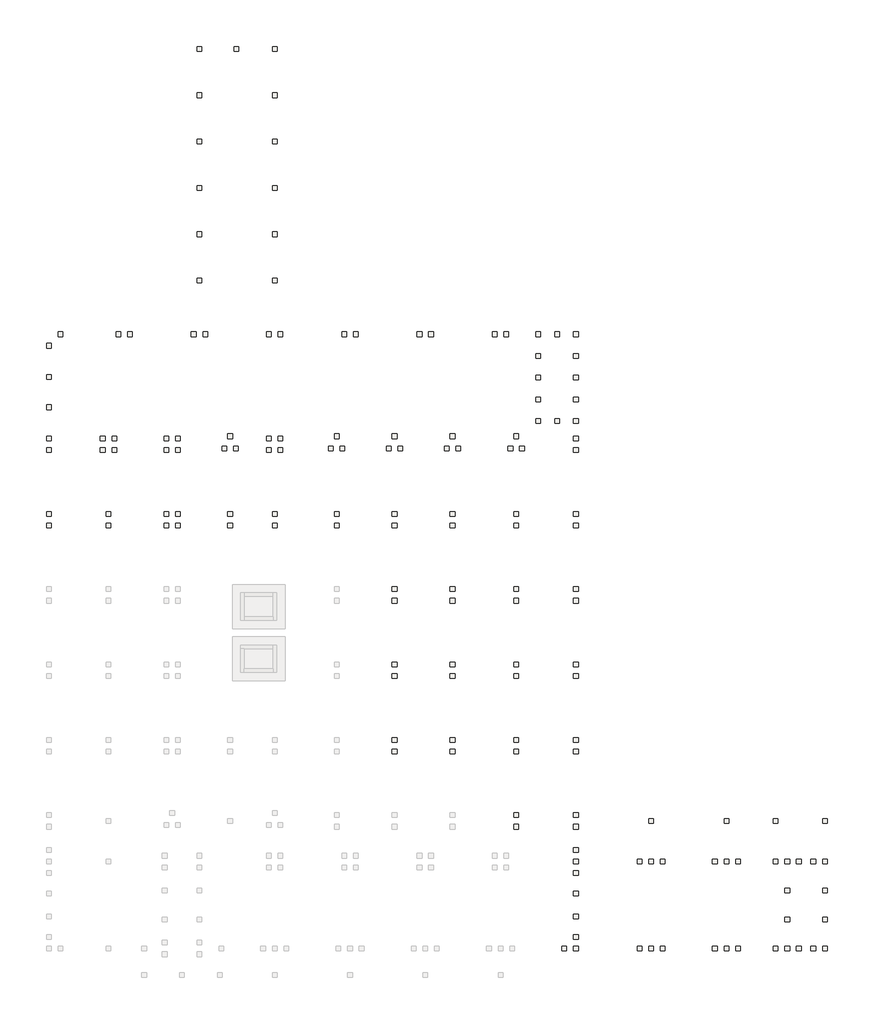
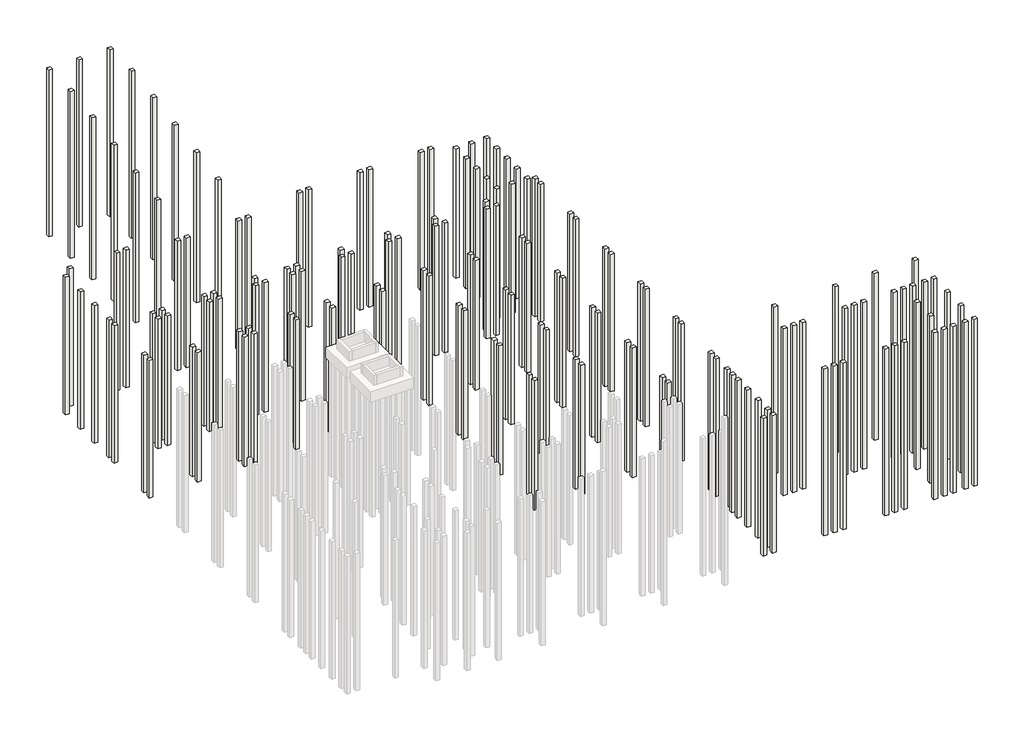
# Not in any storey, part 2 of 2: 160 footings.
# Revit data of these elements (continued)
# Element 4 (IfcFooting, "NLRS_17_SFO_TLB_funderingspaal geheid beton prefab-AV-MMBPC_gen_rsf : heipaal beton prefab_gen__bxh 400x400")
#   IfcGUID = "10$Kfo5uPCAOPJEOo5LEs3"
#   Slanted Angle = 0.00°
#   NLRS_S_draagvermogen_trek = 0.00 kN
#   NLRS_S_draagvermogen_druk = 0.00 kN
#   Angle = 0.00°
#   IsExternal = yes
#   LoadBearing = yes
#   Slanted = 0
#   Phase Created = NLRS_nieuw
#   Materials on its faces: "NLRS_f2_beton prefab_gen_rsf"
# Element 5 (IfcFooting, "NLRS_17_SFO_TLB_funderingspaal geheid beton prefab-AV-MMBPC_gen_rsf : heipaal beton prefab_gen__bxh 400x400")
#   IfcGUID = "10$Kfo5uPCAOPJEOo5LEsU"
#   Slanted Angle = 0.00°
#   NLRS_S_draagvermogen_trek = 0.00 kN
#   NLRS_S_draagvermogen_druk = 0.00 kN
#   Angle = 0.00°
#   IsExternal = yes
#   LoadBearing = yes
#   Slanted = 0
#   Phase Created = NLRS_nieuw
#   Materials on its faces: "NLRS_f2_beton prefab_gen_rsf"
# Element 6 (IfcFooting, "NLRS_17_SFO_TLB_funderingspaal geheid beton prefab-AV-MMBPC_gen_rsf : heipaal beton prefab_gen__bxh 400x400")
#   IfcGUID = "10$Kfo5uPCAOPJEOo5LEsG"
#   Slanted Angle = 0.00°
#   NLRS_S_draagvermogen_trek = 0.00 kN
#   NLRS_S_draagvermogen_druk = 0.00 kN
#   Angle = 0.00°
#   IsExternal = yes
#   LoadBearing = yes
#   Slanted = 0
#   Phase Created = NLRS_nieuw
#   Materials on its faces: "NLRS_f2_beton prefab_gen_rsf"
# Element 7 (IfcFooting, "NLRS_17_SFO_TLB_funderingspaal geheid beton prefab-AV-MMBPC_gen_rsf : heipaal beton prefab_gen__bxh 400x400")
#   IfcGUID = "10$Kfo5uPCAOPJEOo5LEre"
#   Slanted Angle = 0.00°
#   NLRS_S_draagvermogen_trek = 0.00 kN
#   NLRS_S_draagvermogen_druk = 0.00 kN
#   Angle = 0.00°
#   IsExternal = yes
#   LoadBearing = yes
#   Slanted = 0
#   Phase Created = NLRS_nieuw
#   Materials on its faces: "NLRS_f2_beton prefab_gen_rsf"
# Element 8 (IfcFooting, "NLRS_17_SFO_TLB_funderingspaal geheid beton prefab-AV-MMBPC_gen_rsf : heipaal beton prefab_gen__bxh 400x400")
#   IfcGUID = "10$Kfo5uPCAOPJEOo5LErg"
#   Slanted Angle = 0.00°
#   NLRS_S_draagvermogen_trek = 0.00 kN
#   NLRS_S_draagvermogen_druk = 0.00 kN
#   Angle = 0.00°
#   IsExternal = yes
#   LoadBearing = yes
#   Slanted = 0
#   Phase Created = NLRS_nieuw
#   Materials on its faces: "NLRS_f2_beton prefab_gen_rsf"
# Element 9 (IfcFooting, "NLRS_17_SFO_TLB_funderingspaal geheid beton prefab-AV-MMBPC_gen_rsf : heipaal beton prefab_gen__bxh 400x400")
#   IfcGUID = "10$Kfo5uPCAOPJEOo5LEpb"
#   Slanted Angle = 0.00°
#   NLRS_S_draagvermogen_trek = 0.00 kN
#   NLRS_S_draagvermogen_druk = 0.00 kN
#   Angle = 0.00°
#   IsExternal = yes
#   LoadBearing = yes
#   Slanted = 0
#   Phase Created = NLRS_nieuw
#   Materials on its faces: "NLRS_f2_beton prefab_gen_rsf"
# Element 10 (IfcFooting, "NLRS_17_SFO_TLB_funderingspaal geheid beton prefab-AV-MMBPC_gen_rsf : heipaal beton prefab_gen__bxh 400x400")
#   IfcGUID = "10$Kfo5uPCAOPJEOo5LEpd"
#   Slanted Angle = 0.00°
#   NLRS_S_draagvermogen_trek = 0.00 kN
#   NLRS_S_draagvermogen_druk = 0.00 kN
#   Angle = 0.00°
#   IsExternal = yes
#   LoadBearing = yes
#   Slanted = 0
#   Phase Created = NLRS_nieuw
#   Materials on its faces: "NLRS_f2_beton prefab_gen_rsf"
# Element 11 (IfcFooting, "NLRS_17_SFO_TLB_funderingspaal geheid beton prefab-AV-MMBPC_gen_rsf : heipaal beton prefab_gen__bxh 400x400")
#   IfcGUID = "10$Kfo5uPCAOPJEOo5LEpz"
#   Slanted Angle = 0.00°
#   NLRS_S_draagvermogen_trek = 0.00 kN
#   NLRS_S_draagvermogen_druk = 0.00 kN
#   Angle = 0.00°
#   IsExternal = yes
#   LoadBearing = yes
#   Slanted = 0
#   Phase Created = NLRS_nieuw
#   Materials on its faces: "NLRS_f2_beton prefab_gen_rsf"
# Element 12 (IfcFooting, "NLRS_17_SFO_TLB_funderingspaal geheid beton prefab-AV-MMBPC_gen_rsf : heipaal beton prefab_gen__bxh 400x400")
#   IfcGUID = "10$Kfo5uPCAOPJEOo5LEp$"
#   Slanted Angle = 0.00°
#   NLRS_S_draagvermogen_trek = 0.00 kN
#   NLRS_S_draagvermogen_druk = 0.00 kN
#   Angle = 0.00°
#   IsExternal = yes
#   LoadBearing = yes
#   Slanted = 0
#   Phase Created = NLRS_nieuw
#   Materials on its faces: "NLRS_f2_beton prefab_gen_rsf"
# Element 13 (IfcFooting, "NLRS_17_SFO_TLB_funderingspaal geheid beton prefab-AV-MMBPC_gen_rsf : heipaal beton prefab_gen__bxh 400x400")
#   IfcGUID = "10$Kfo5uPCAOPJEOo5LFTh"
#   Slanted Angle = 0.00°
#   NLRS_S_draagvermogen_trek = 0.00 kN
#   NLRS_S_draagvermogen_druk = 0.00 kN
#   Angle = 0.00°
#   IsExternal = yes
#   LoadBearing = yes
#   Slanted = 0
#   Phase Created = NLRS_nieuw
#   Materials on its faces: "NLRS_f2_beton prefab_gen_rsf"
# Element 14 (IfcFooting, "NLRS_17_SFO_TLB_funderingspaal geheid beton prefab-AV-MMBPC_gen_rsf : heipaal beton prefab_gen__bxh 400x400")
#   IfcGUID = "10$Kfo5uPCAOPJEOo5LFSD"
#   Slanted Angle = 0.00°
#   NLRS_S_draagvermogen_trek = 0.00 kN
#   NLRS_S_draagvermogen_druk = 0.00 kN
#   Angle = 0.00°
#   IsExternal = yes
#   LoadBearing = yes
#   Slanted = 0
#   Phase Created = NLRS_nieuw
#   Materials on its faces: "NLRS_f2_beton prefab_gen_rsf"
# Element 15 (IfcFooting, "NLRS_17_SFO_TLB_funderingspaal geheid beton prefab-AV-MMBPC_gen_rsf : heipaal beton prefab_gen__bxh 400x400")
#   IfcGUID = "10$Kfo5uPCAOPJEOo5LFSk"
#   Slanted Angle = 0.00°
#   NLRS_S_draagvermogen_trek = 0.00 kN
#   NLRS_S_draagvermogen_druk = 0.00 kN
#   Angle = 0.00°
#   IsExternal = yes
#   LoadBearing = yes
#   Slanted = 0
#   Phase Created = NLRS_nieuw
#   Materials on its faces: "NLRS_f2_beton prefab_gen_rsf"
# Element 16 (IfcFooting, "NLRS_17_SFO_TLB_funderingspaal geheid beton prefab-AV-MMBPC_gen_rsf : heipaal beton prefab_gen__bxh 400x400")
#   IfcGUID = "10$Kfo5uPCAOPJEOo5LFSv"
#   Slanted Angle = 0.00°
#   NLRS_S_draagvermogen_trek = 0.00 kN
#   NLRS_S_draagvermogen_druk = 0.00 kN
#   Angle = 0.00°
#   IsExternal = yes
#   LoadBearing = yes
#   Slanted = 0
#   Phase Created = NLRS_nieuw
#   Materials on its faces: "NLRS_f2_beton prefab_gen_rsf"
# Element 17 (IfcFooting, "NLRS_17_SFO_TLB_funderingspaal geheid beton prefab-AV-MMBPC_gen_rsf : heipaal beton prefab_gen__bxh 400x400")
#   IfcGUID = "10$Kfo5uPCAOPJEOo5LFSs"
#   Slanted Angle = 0.00°
#   NLRS_S_draagvermogen_trek = 0.00 kN
#   NLRS_S_draagvermogen_druk = 0.00 kN
#   Angle = 0.00°
#   IsExternal = yes
#   LoadBearing = yes
#   Slanted = 0
#   Phase Created = NLRS_nieuw
#   Materials on its faces: "NLRS_f2_beton prefab_gen_rsf"
# Element 18 (IfcFooting, "NLRS_17_SFO_TLB_funderingspaal geheid beton prefab-AV-MMBPC_gen_rsf : heipaal beton prefab_gen__bxh 400x400")
#   IfcGUID = "10$Kfo5uPCAOPJEOo5LFR1"
#   Slanted Angle = 0.00°
#   NLRS_S_draagvermogen_trek = 0.00 kN
#   NLRS_S_draagvermogen_druk = 0.00 kN
#   Angle = 0.00°
#   IsExternal = yes
#   LoadBearing = yes
#   Slanted = 0
#   Phase Created = NLRS_nieuw
#   Materials on its faces: "NLRS_f2_beton prefab_gen_rsf"
# Element 19 (IfcFooting, "NLRS_17_SFO_TLB_funderingspaal geheid beton prefab-AV-MMBPC_gen_rsf : heipaal beton prefab_gen__bxh 400x400")
#   IfcGUID = "10$Kfo5uPCAOPJEOo5LFQO"
#   Slanted Angle = 0.00°
#   NLRS_S_draagvermogen_trek = 0.00 kN
#   NLRS_S_draagvermogen_druk = 0.00 kN
#   Angle = 0.00°
#   IsExternal = yes
#   LoadBearing = yes
#   Slanted = 0
#   Phase Created = NLRS_nieuw
#   Materials on its faces: "NLRS_f2_beton prefab_gen_rsf"
# Element 20 (IfcFooting, "NLRS_17_SFO_TLB_funderingspaal geheid beton prefab-AV-MMBPC_gen_rsf : heipaal beton prefab_gen__bxh 400x400")
#   IfcGUID = "10$Kfo5uPCAOPJEOo5LFQJ"
#   Slanted Angle = 0.00°
#   NLRS_S_draagvermogen_trek = 0.00 kN
#   NLRS_S_draagvermogen_druk = 0.00 kN
#   Angle = 0.00°
#   IsExternal = yes
#   LoadBearing = yes
#   Slanted = 0
#   Phase Created = NLRS_nieuw
#   Materials on its faces: "NLRS_f2_beton prefab_gen_rsf"
# Element 21 (IfcFooting, "NLRS_17_SFO_TLB_funderingspaal geheid beton prefab-AV-MMBPC_gen_rsf : heipaal beton prefab_gen__bxh 400x400")
#   IfcGUID = "10$Kfo5uPCAOPJEOo5LFQk"
#   Slanted Angle = 0.00°
#   NLRS_S_draagvermogen_trek = 0.00 kN
#   NLRS_S_draagvermogen_druk = 0.00 kN
#   Angle = 0.00°
#   IsExternal = yes
#   LoadBearing = yes
#   Slanted = 0
#   Phase Created = NLRS_nieuw
#   Materials on its faces: "NLRS_f2_beton prefab_gen_rsf"
# Element 22 (IfcFooting, "NLRS_17_SFO_TLB_funderingspaal geheid beton prefab-AV-MMBPC_gen_rsf : heipaal beton prefab_gen__bxh 400x400")
#   IfcGUID = "10$Kfo5uPCAOPJEOo5LFPx"
#   Slanted Angle = 0.00°
#   NLRS_S_draagvermogen_trek = 0.00 kN
#   NLRS_S_draagvermogen_druk = 0.00 kN
#   Angle = 0.00°
#   IsExternal = yes
#   LoadBearing = yes
#   Slanted = 0
#   Phase Created = NLRS_nieuw
#   Materials on its faces: "NLRS_f2_beton prefab_gen_rsf"
# Element 23 (IfcFooting, "NLRS_17_SFO_TLB_funderingspaal geheid beton prefab-AV-MMBPC_gen_rsf : heipaal beton prefab_gen__bxh 400x400")
#   IfcGUID = "10$Kfo5uPCAOPJEOo5LFOK"
#   Slanted Angle = 0.00°
#   NLRS_S_draagvermogen_trek = 0.00 kN
#   NLRS_S_draagvermogen_druk = 0.00 kN
#   Angle = 0.00°
#   IsExternal = yes
#   LoadBearing = yes
#   Slanted = 0
#   Phase Created = NLRS_nieuw
#   Materials on its faces: "NLRS_f2_beton prefab_gen_rsf"
# Element 24 (IfcFooting, "NLRS_17_SFO_TLB_funderingspaal geheid beton prefab-AV-MMBPC_gen_rsf : heipaal beton prefab_gen__bxh 400x400")
#   IfcGUID = "10$Kfo5uPCAOPJEOo5LFOl"
#   Slanted Angle = 0.00°
#   NLRS_S_draagvermogen_trek = 0.00 kN
#   NLRS_S_draagvermogen_druk = 0.00 kN
#   Angle = 0.00°
#   IsExternal = yes
#   LoadBearing = yes
#   Slanted = 0
#   Phase Created = NLRS_nieuw
#   Materials on its faces: "NLRS_f2_beton prefab_gen_rsf"
# Element 25 (IfcFooting, "NLRS_17_SFO_TLB_funderingspaal geheid beton prefab-AV-MMBPC_gen_rsf : heipaal beton prefab_gen__bxh 400x400")
#   IfcGUID = "3loy75XKz2Rw4dS8JWiamE"
#   Slanted Angle = 0.00°
#   NLRS_S_draagvermogen_trek = 0.00 kN
#   NLRS_S_draagvermogen_druk = 0.00 kN
#   Angle = 0.00°
#   IsExternal = yes
#   LoadBearing = yes
#   Slanted = 0
#   Phase Created = NLRS_nieuw
#   Materials on its faces: "NLRS_f2_beton prefab_gen_rsf"
# Element 26 (IfcFooting, "NLRS_17_SFO_TLB_funderingspaal geheid beton prefab-AV-MMBPC_gen_rsf : heipaal beton prefab_gen__bxh 400x400")
#   IfcGUID = "3loy75XKz2Rw4dS8JWiamC"
#   Slanted Angle = 0.00°
#   NLRS_S_draagvermogen_trek = 0.00 kN
#   NLRS_S_draagvermogen_druk = 0.00 kN
#   Angle = 0.00°
#   IsExternal = yes
#   LoadBearing = yes
#   Slanted = 0
#   Phase Created = NLRS_nieuw
#   Materials on its faces: "NLRS_f2_beton prefab_gen_rsf"
# Element 27 (IfcFooting, "NLRS_17_SFO_TLB_funderingspaal geheid beton prefab-AV-MMBPC_gen_rsf : heipaal beton prefab_gen__bxh 400x400")
#   IfcGUID = "3loy75XKz2Rw4dS8JWiamv"
#   Slanted Angle = 0.00°
#   NLRS_S_draagvermogen_trek = 0.00 kN
#   NLRS_S_draagvermogen_druk = 0.00 kN
#   Angle = 0.00°
#   IsExternal = yes
#   LoadBearing = yes
#   Slanted = 0
#   Phase Created = NLRS_nieuw
#   Materials on its faces: "NLRS_f2_beton prefab_gen_rsf"
# Element 28 (IfcFooting, "NLRS_17_SFO_TLB_funderingspaal geheid beton prefab-AV-MMBPC_gen_rsf : heipaal beton prefab_gen__bxh 400x400")
#   IfcGUID = "3loy75XKz2Rw4dS8JWiam$"
#   Slanted Angle = 0.00°
#   NLRS_S_draagvermogen_trek = 0.00 kN
#   NLRS_S_draagvermogen_druk = 0.00 kN
#   Angle = 0.00°
#   IsExternal = yes
#   LoadBearing = yes
#   Slanted = 0
#   Phase Created = NLRS_nieuw
#   Materials on its faces: "NLRS_f2_beton prefab_gen_rsf"
# Element 29 (IfcFooting, "NLRS_17_SFO_TLB_funderingspaal geheid beton prefab-AV-MMBPC_gen_rsf : heipaal beton prefab_gen__bxh 400x400")
#   IfcGUID = "3loy75XKz2Rw4dS8JWiama"
#   Slanted Angle = 0.00°
#   NLRS_S_draagvermogen_trek = 0.00 kN
#   NLRS_S_draagvermogen_druk = 0.00 kN
#   Angle = 0.00°
#   IsExternal = yes
#   LoadBearing = yes
#   Slanted = 0
#   Phase Created = NLRS_nieuw
#   Materials on its faces: "NLRS_f2_beton prefab_gen_rsf"
# Element 30 (IfcFooting, "NLRS_17_SFO_TLB_funderingspaal geheid beton prefab-AV-MMBPC_gen_rsf : heipaal beton prefab_gen__bxh 400x400")
#   IfcGUID = "3loy75XKz2Rw4dS8JWiamg"
#   Slanted Angle = 0.00°
#   NLRS_S_draagvermogen_trek = 0.00 kN
#   NLRS_S_draagvermogen_druk = 0.00 kN
#   Angle = 0.00°
#   IsExternal = yes
#   LoadBearing = yes
#   Slanted = 0
#   Phase Created = NLRS_nieuw
#   Materials on its faces: "NLRS_f2_beton prefab_gen_rsf"
# Element 31 (IfcFooting, "NLRS_17_SFO_TLB_funderingspaal geheid beton prefab-AV-MMBPC_gen_rsf : heipaal beton prefab_gen__bxh 400x400")
#   IfcGUID = "3loy75XKz2Rw4dS8JWiapN"
#   Slanted Angle = 0.00°
#   NLRS_S_draagvermogen_trek = 0.00 kN
#   NLRS_S_draagvermogen_druk = 0.00 kN
#   Angle = 0.00°
#   IsExternal = yes
#   LoadBearing = yes
#   Slanted = 0
#   Phase Created = NLRS_nieuw
#   Materials on its faces: "NLRS_f2_beton prefab_gen_rsf"
# Element 32 (IfcFooting, "NLRS_17_SFO_TLB_funderingspaal geheid beton prefab-AV-MMBPC_gen_rsf : heipaal beton prefab_gen__bxh 400x400")
#   IfcGUID = "3loy75XKz2Rw4dS8JWiapL"
#   Slanted Angle = 0.00°
#   NLRS_S_draagvermogen_trek = 0.00 kN
#   NLRS_S_draagvermogen_druk = 0.00 kN
#   Angle = 0.00°
#   IsExternal = yes
#   LoadBearing = yes
#   Slanted = 0
#   Phase Created = NLRS_nieuw
#   Materials on its faces: "NLRS_f2_beton prefab_gen_rsf"
# Element 33 (IfcFooting, "NLRS_17_SFO_TLB_funderingspaal geheid beton prefab-AV-MMBPC_gen_rsf : heipaal beton prefab_gen__bxh 400x400")
#   IfcGUID = "3loy75XKz2Rw4dS8JWiap2"
#   Slanted Angle = 0.00°
#   NLRS_S_draagvermogen_trek = 0.00 kN
#   NLRS_S_draagvermogen_druk = 0.00 kN
#   Angle = 0.00°
#   IsExternal = yes
#   LoadBearing = yes
#   Slanted = 0
#   Phase Created = NLRS_nieuw
#   Materials on its faces: "NLRS_f2_beton prefab_gen_rsf"
# Element 34 (IfcFooting, "NLRS_17_SFO_TLB_funderingspaal geheid beton prefab-AV-MMBPC_gen_rsf : heipaal beton prefab_gen__bxh 400x400")
#   IfcGUID = "3loy75XKz2Rw4dS8JWiap0"
#   Slanted Angle = 0.00°
#   NLRS_S_draagvermogen_trek = 0.00 kN
#   NLRS_S_draagvermogen_druk = 0.00 kN
#   Angle = 0.00°
#   IsExternal = yes
#   LoadBearing = yes
#   Slanted = 0
#   Phase Created = NLRS_nieuw
#   Materials on its faces: "NLRS_f2_beton prefab_gen_rsf"
# Element 35 (IfcFooting, "NLRS_17_SFO_TLB_funderingspaal geheid beton prefab-AV-MMBPC_gen_rsf : heipaal beton prefab_gen__bxh 400x400")
#   IfcGUID = "3loy75XKz2Rw4dS8JWiapD"
#   Slanted Angle = 0.00°
#   NLRS_S_draagvermogen_trek = 0.00 kN
#   NLRS_S_draagvermogen_druk = 0.00 kN
#   Angle = 0.00°
#   IsExternal = yes
#   LoadBearing = yes
#   Slanted = 0
#   Phase Created = NLRS_nieuw
#   Materials on its faces: "NLRS_f2_beton prefab_gen_rsf"
# Element 36 (IfcFooting, "NLRS_17_SFO_TLB_funderingspaal geheid beton prefab-AV-MMBPC_gen_rsf : heipaal beton prefab_gen__bxh 400x400")
#   IfcGUID = "3loy75XKz2Rw4dS8JWiapp"
#   Slanted Angle = 0.00°
#   NLRS_S_draagvermogen_trek = 0.00 kN
#   NLRS_S_draagvermogen_druk = 0.00 kN
#   Angle = 0.00°
#   IsExternal = yes
#   LoadBearing = yes
#   Slanted = 0
#   Phase Created = NLRS_nieuw
#   Materials on its faces: "NLRS_f2_beton prefab_gen_rsf"
# Element 37 (IfcFooting, "NLRS_17_SFO_TLB_funderingspaal geheid beton prefab-AV-MMBPC_gen_rsf : heipaal beton prefab_gen__bxh 400x400")
#   IfcGUID = "3loy75XKz2Rw4dS8JWiao6"
#   Slanted Angle = 0.00°
#   NLRS_S_draagvermogen_trek = 0.00 kN
#   NLRS_S_draagvermogen_druk = 0.00 kN
#   Angle = 0.00°
#   IsExternal = yes
#   LoadBearing = yes
#   Slanted = 0
#   Phase Created = NLRS_nieuw
#   Materials on its faces: "NLRS_f2_beton prefab_gen_rsf"
# Element 38 (IfcFooting, "NLRS_17_SFO_TLB_funderingspaal geheid beton prefab-AV-MMBPC_gen_rsf : heipaal beton prefab_gen__bxh 400x400")
#   IfcGUID = "3loy75XKz2Rw4dS8JWiao4"
#   Slanted Angle = 0.00°
#   NLRS_S_draagvermogen_trek = 0.00 kN
#   NLRS_S_draagvermogen_druk = 0.00 kN
#   Angle = 0.00°
#   IsExternal = yes
#   LoadBearing = yes
#   Slanted = 0
#   Phase Created = NLRS_nieuw
#   Materials on its faces: "NLRS_f2_beton prefab_gen_rsf"
# Element 39 (IfcFooting, "NLRS_17_SFO_TLB_funderingspaal geheid beton prefab-AV-MMBPC_gen_rsf : heipaal beton prefab_gen__bxh 400x400")
#   IfcGUID = "3loy75XKz2Rw4dS8JWiaon"
#   Slanted Angle = 0.00°
#   NLRS_S_draagvermogen_trek = 0.00 kN
#   NLRS_S_draagvermogen_druk = 0.00 kN
#   Angle = 0.00°
#   IsExternal = yes
#   LoadBearing = yes
#   Slanted = 0
#   Phase Created = NLRS_nieuw
#   Materials on its faces: "NLRS_f2_beton prefab_gen_rsf"
# Element 40 (IfcFooting, "NLRS_17_SFO_TLB_funderingspaal geheid beton prefab-AV-MMBPC_gen_rsf : heipaal beton prefab_gen__bxh 400x400")
#   IfcGUID = "3loy75XKz2Rw4dS8JWiaot"
#   Slanted Angle = 0.00°
#   NLRS_S_draagvermogen_trek = 0.00 kN
#   NLRS_S_draagvermogen_druk = 0.00 kN
#   Angle = 0.00°
#   IsExternal = yes
#   LoadBearing = yes
#   Slanted = 0
#   Phase Created = NLRS_nieuw
#   Materials on its faces: "NLRS_f2_beton prefab_gen_rsf"
# Element 41 (IfcFooting, "NLRS_17_SFO_TLB_funderingspaal geheid beton prefab-AV-MMBPC_gen_rsf : heipaal beton prefab_gen__bxh 400x400")
#   IfcGUID = "3loy75XKz2Rw4dS8JWiaoy"
#   Slanted Angle = 0.00°
#   NLRS_S_draagvermogen_trek = 0.00 kN
#   NLRS_S_draagvermogen_druk = 0.00 kN
#   Angle = 0.00°
#   IsExternal = yes
#   LoadBearing = yes
#   Slanted = 0
#   Phase Created = NLRS_nieuw
#   Materials on its faces: "NLRS_f2_beton prefab_gen_rsf"
# Element 42 (IfcFooting, "NLRS_17_SFO_TLB_funderingspaal geheid beton prefab-AV-MMBPC_gen_rsf : heipaal beton prefab_gen__bxh 400x400")
#   IfcGUID = "3loy75XKz2Rw4dS8JWiaoY"
#   Slanted Angle = 0.00°
#   NLRS_S_draagvermogen_trek = 0.00 kN
#   NLRS_S_draagvermogen_druk = 0.00 kN
#   Angle = 0.00°
#   IsExternal = yes
#   LoadBearing = yes
#   Slanted = 0
#   Phase Created = NLRS_nieuw
#   Materials on its faces: "NLRS_f2_beton prefab_gen_rsf"
# Element 43 (IfcFooting, "NLRS_17_SFO_TLB_funderingspaal geheid beton prefab-AV-MMBPC_gen_rsf : heipaal beton prefab_gen__bxh 400x400")
#   IfcGUID = "3loy75XKz2Rw4dS8JWiaol"
#   Slanted Angle = 0.00°
#   NLRS_S_draagvermogen_trek = 0.00 kN
#   NLRS_S_draagvermogen_druk = 0.00 kN
#   Angle = 0.00°
#   IsExternal = yes
#   LoadBearing = yes
#   Slanted = 0
#   Phase Created = NLRS_nieuw
#   Materials on its faces: "NLRS_f2_beton prefab_gen_rsf"
# Element 44 (IfcFooting, "NLRS_17_SFO_TLB_funderingspaal geheid beton prefab-AV-MMBPC_gen_rsf : heipaal beton prefab_gen__bxh 400x400")
#   IfcGUID = "3loy75XKz2Rw4dS8JWiaoj"
#   Slanted Angle = 0.00°
#   NLRS_S_draagvermogen_trek = 0.00 kN
#   NLRS_S_draagvermogen_druk = 0.00 kN
#   Angle = 0.00°
#   IsExternal = yes
#   LoadBearing = yes
#   Slanted = 0
#   Phase Created = NLRS_nieuw
#   Materials on its faces: "NLRS_f2_beton prefab_gen_rsf"
# Element 45 (IfcFooting, "NLRS_17_SFO_TLB_funderingspaal geheid beton prefab-AV-MMBPC_gen_rsf : heipaal beton prefab_gen__bxh 400x400")
#   IfcGUID = "3loy75XKz2Rw4dS8JWiarQ"
#   Slanted Angle = 0.00°
#   NLRS_S_draagvermogen_trek = 0.00 kN
#   NLRS_S_draagvermogen_druk = 0.00 kN
#   Angle = 0.00°
#   IsExternal = yes
#   LoadBearing = yes
#   Slanted = 0
#   Phase Created = NLRS_nieuw
#   Materials on its faces: "NLRS_f2_beton prefab_gen_rsf"
# Element 46 (IfcFooting, "NLRS_17_SFO_TLB_funderingspaal geheid beton prefab-AV-MMBPC_gen_rsf : heipaal beton prefab_gen__bxh 400x400")
#   IfcGUID = "3loy75XKz2Rw4dS8JWiarO"
#   Slanted Angle = 0.00°
#   NLRS_S_draagvermogen_trek = 0.00 kN
#   NLRS_S_draagvermogen_druk = 0.00 kN
#   Angle = 0.00°
#   IsExternal = yes
#   LoadBearing = yes
#   Slanted = 0
#   Phase Created = NLRS_nieuw
#   Materials on its faces: "NLRS_f2_beton prefab_gen_rsf"
# Element 47 (IfcFooting, "NLRS_17_SFO_TLB_funderingspaal geheid beton prefab-AV-MMBPC_gen_rsf : heipaal beton prefab_gen__bxh 400x400")
#   IfcGUID = "3loy75XKz2Rw4dS8JWiar5"
#   Slanted Angle = 0.00°
#   NLRS_S_draagvermogen_trek = 0.00 kN
#   NLRS_S_draagvermogen_druk = 0.00 kN
#   Angle = 0.00°
#   IsExternal = yes
#   LoadBearing = yes
#   Slanted = 0
#   Phase Created = NLRS_nieuw
#   Materials on its faces: "NLRS_f2_beton prefab_gen_rsf"
# Element 48 (IfcFooting, "NLRS_17_SFO_TLB_funderingspaal geheid beton prefab-AV-MMBPC_gen_rsf : heipaal beton prefab_gen__bxh 400x400")
#   IfcGUID = "3loy75XKz2Rw4dS8JWiarB"
#   Slanted Angle = 0.00°
#   NLRS_S_draagvermogen_trek = 0.00 kN
#   NLRS_S_draagvermogen_druk = 0.00 kN
#   Angle = 0.00°
#   IsExternal = yes
#   LoadBearing = yes
#   Slanted = 0
#   Phase Created = NLRS_nieuw
#   Materials on its faces: "NLRS_f2_beton prefab_gen_rsf"
# Element 49 (IfcFooting, "NLRS_17_SFO_TLB_funderingspaal geheid beton prefab-AV-MMBPC_gen_rsf : heipaal beton prefab_gen__bxh 400x400")
#   IfcGUID = "3loy75XKz2Rw4dS8JWiarm"
#   Slanted Angle = 0.00°
#   NLRS_S_draagvermogen_trek = 0.00 kN
#   NLRS_S_draagvermogen_druk = 0.00 kN
#   Angle = 0.00°
#   IsExternal = yes
#   LoadBearing = yes
#   Slanted = 0
#   Phase Created = NLRS_nieuw
#   Materials on its faces: "NLRS_f2_beton prefab_gen_rsf"
# Element 50 (IfcFooting, "NLRS_17_SFO_TLB_funderingspaal geheid beton prefab-AV-MMBPC_gen_rsf : heipaal beton prefab_gen__bxh 400x400")
#   IfcGUID = "3loy75XKz2Rw4dS8JWiars"
#   Slanted Angle = 0.00°
#   NLRS_S_draagvermogen_trek = 0.00 kN
#   NLRS_S_draagvermogen_druk = 0.00 kN
#   Angle = 0.00°
#   IsExternal = yes
#   LoadBearing = yes
#   Slanted = 0
#   Phase Created = NLRS_nieuw
#   Materials on its faces: "NLRS_f2_beton prefab_gen_rsf"
# Element 51 (IfcFooting, "NLRS_17_SFO_TLB_funderingspaal geheid beton prefab-AV-MMBPC_gen_rsf : heipaal beton prefab_gen__bxh 400x400")
#   IfcGUID = "3loy75XKz2Rw4dS8JWia96"
#   Slanted Angle = 0.00°
#   NLRS_S_draagvermogen_trek = 0.00 kN
#   NLRS_S_draagvermogen_druk = 0.00 kN
#   Angle = 0.00°
#   IsExternal = yes
#   LoadBearing = yes
#   Slanted = 0
#   Phase Created = NLRS_nieuw
#   Materials on its faces: "NLRS_f2_beton prefab_gen_rsf"
# Element 52 (IfcFooting, "NLRS_17_SFO_TLB_funderingspaal geheid beton prefab-AV-MMBPC_gen_rsf : heipaal beton prefab_gen__bxh 400x400")
#   IfcGUID = "3loy75XKz2Rw4dS8JWia94"
#   Slanted Angle = 0.00°
#   NLRS_S_draagvermogen_trek = 0.00 kN
#   NLRS_S_draagvermogen_druk = 0.00 kN
#   Angle = 0.00°
#   IsExternal = yes
#   LoadBearing = yes
#   Slanted = 0
#   Phase Created = NLRS_nieuw
#   Materials on its faces: "NLRS_f2_beton prefab_gen_rsf"
# Element 53 (IfcFooting, "NLRS_17_SFO_TLB_funderingspaal geheid beton prefab-AV-MMBPC_gen_rsf : heipaal beton prefab_gen__bxh 400x400")
#   IfcGUID = "3loy75XKz2Rw4dS8JWia9A"
#   Slanted Angle = 0.00°
#   NLRS_S_draagvermogen_trek = 0.00 kN
#   NLRS_S_draagvermogen_druk = 0.00 kN
#   Angle = 0.00°
#   IsExternal = yes
#   LoadBearing = yes
#   Slanted = 0
#   Phase Created = NLRS_nieuw
#   Materials on its faces: "NLRS_f2_beton prefab_gen_rsf"
# Element 54 (IfcFooting, "NLRS_17_SFO_TLB_funderingspaal geheid beton prefab-AV-MMBPC_gen_rsf : heipaal beton prefab_gen__bxh 400x400")
#   IfcGUID = "3loy75XKz2Rw4dS8JWia98"
#   Slanted Angle = 0.00°
#   NLRS_S_draagvermogen_trek = 0.00 kN
#   NLRS_S_draagvermogen_druk = 0.00 kN
#   Angle = 0.00°
#   IsExternal = yes
#   LoadBearing = yes
#   Slanted = 0
#   Phase Created = NLRS_nieuw
#   Materials on its faces: "NLRS_f2_beton prefab_gen_rsf"
# Element 55 (IfcFooting, "NLRS_17_SFO_TLB_funderingspaal geheid beton prefab-AV-MMBPC_gen_rsf : heipaal beton prefab_gen__bxh 400x400")
#   IfcGUID = "3loy75XKz2Rw4dS8JWia9l"
#   Slanted Angle = 0.00°
#   NLRS_S_draagvermogen_trek = 0.00 kN
#   NLRS_S_draagvermogen_druk = 0.00 kN
#   Angle = 0.00°
#   IsExternal = yes
#   LoadBearing = yes
#   Slanted = 0
#   Phase Created = NLRS_nieuw
#   Materials on its faces: "NLRS_f2_beton prefab_gen_rsf"
# Element 56 (IfcFooting, "NLRS_17_SFO_TLB_funderingspaal geheid beton prefab-AV-MMBPC_gen_rsf : heipaal beton prefab_gen__bxh 400x400")
#   IfcGUID = "3loy75XKz2Rw4dS8JWia9j"
#   Slanted Angle = 0.00°
#   NLRS_S_draagvermogen_trek = 0.00 kN
#   NLRS_S_draagvermogen_druk = 0.00 kN
#   Angle = 0.00°
#   IsExternal = yes
#   LoadBearing = yes
#   Slanted = 0
#   Phase Created = NLRS_nieuw
#   Materials on its faces: "NLRS_f2_beton prefab_gen_rsf"
# Element 57 (IfcFooting, "NLRS_17_SFO_TLB_funderingspaal geheid beton prefab-AV-MMBPC_gen_rsf : heipaal beton prefab_gen__bxh 400x400")
#   IfcGUID = "3loy75XKz2Rw4dS8JWia8J"
#   Slanted Angle = 0.00°
#   NLRS_S_draagvermogen_trek = 0.00 kN
#   NLRS_S_draagvermogen_druk = 0.00 kN
#   Angle = 0.00°
#   IsExternal = yes
#   LoadBearing = yes
#   Slanted = 0
#   Phase Created = NLRS_nieuw
#   Materials on its faces: "NLRS_f2_beton prefab_gen_rsf"
# Element 58 (IfcFooting, "NLRS_17_SFO_TLB_funderingspaal geheid beton prefab-AV-MMBPC_gen_rsf : heipaal beton prefab_gen__bxh 400x400")
#   IfcGUID = "3loy75XKz2Rw4dS8JWia8H"
#   Slanted Angle = 0.00°
#   NLRS_S_draagvermogen_trek = 0.00 kN
#   NLRS_S_draagvermogen_druk = 0.00 kN
#   Angle = 0.00°
#   IsExternal = yes
#   LoadBearing = yes
#   Slanted = 0
#   Phase Created = NLRS_nieuw
#   Materials on its faces: "NLRS_f2_beton prefab_gen_rsf"
# Element 59 (IfcFooting, "NLRS_17_SFO_TLB_funderingspaal geheid beton prefab-AV-MMBPC_gen_rsf : heipaal beton prefab_gen__bxh 400x400")
#   IfcGUID = "3loy75XKz2Rw4dS8JWia8q"
#   Slanted Angle = 0.00°
#   NLRS_S_draagvermogen_trek = 0.00 kN
#   NLRS_S_draagvermogen_druk = 0.00 kN
#   Angle = 0.00°
#   IsExternal = yes
#   LoadBearing = yes
#   Slanted = 0
#   Phase Created = NLRS_nieuw
#   Materials on its faces: "NLRS_f2_beton prefab_gen_rsf"
# Element 60 (IfcFooting, "NLRS_17_SFO_TLB_funderingspaal geheid beton prefab-AV-MMBPC_gen_rsf : heipaal beton prefab_gen__bxh 400x400")
#   IfcGUID = "3loy75XKz2Rw4dS8JWia8w"
#   Slanted Angle = 0.00°
#   NLRS_S_draagvermogen_trek = 0.00 kN
#   NLRS_S_draagvermogen_druk = 0.00 kN
#   Angle = 0.00°
#   IsExternal = yes
#   LoadBearing = yes
#   Slanted = 0
#   Phase Created = NLRS_nieuw
#   Materials on its faces: "NLRS_f2_beton prefab_gen_rsf"
# Element 61 (IfcFooting, "NLRS_17_SFO_TLB_funderingspaal geheid beton prefab-AV-MMBPC_gen_rsf : heipaal beton prefab_gen__bxh 400x400")
#   IfcGUID = "3loy75XKz2Rw4dS8JWia8u"
#   Slanted Angle = 0.00°
#   NLRS_S_draagvermogen_trek = 0.00 kN
#   NLRS_S_draagvermogen_druk = 0.00 kN
#   Angle = 0.00°
#   IsExternal = yes
#   LoadBearing = yes
#   Slanted = 0
#   Phase Created = NLRS_nieuw
#   Materials on its faces: "NLRS_f2_beton prefab_gen_rsf"
# Element 62 (IfcFooting, "NLRS_17_SFO_TLB_funderingspaal geheid beton prefab-AV-MMBPC_gen_rsf : heipaal beton prefab_gen__bxh 400x400")
#   IfcGUID = "3loy75XKz2Rw4dS8JWiaDh"
#   Slanted Angle = 0.00°
#   NLRS_S_draagvermogen_trek = 0.00 kN
#   NLRS_S_draagvermogen_druk = 0.00 kN
#   Angle = 0.00°
#   IsExternal = yes
#   LoadBearing = yes
#   Slanted = 0
#   Phase Created = NLRS_nieuw
#   Materials on its faces: "NLRS_f2_beton prefab_gen_rsf"
# Element 63 (IfcFooting, "NLRS_17_SFO_TLB_funderingspaal geheid beton prefab-AV-MMBPC_gen_rsf : heipaal beton prefab_gen__bxh 400x400")
#   IfcGUID = "3loy75XKz2Rw4dS8JWiaDf"
#   Slanted Angle = 0.00°
#   NLRS_S_draagvermogen_trek = 0.00 kN
#   NLRS_S_draagvermogen_druk = 0.00 kN
#   Angle = 0.00°
#   IsExternal = yes
#   LoadBearing = yes
#   Slanted = 0
#   Phase Created = NLRS_nieuw
#   Materials on its faces: "NLRS_f2_beton prefab_gen_rsf"
# Element 64 (IfcFooting, "NLRS_17_SFO_TLB_funderingspaal geheid beton prefab-AV-MMBPC_gen_rsf : heipaal beton prefab_gen__bxh 400x400")
#   IfcGUID = "3loy75XKz2Rw4dS8JWiaDl"
#   Slanted Angle = 0.00°
#   NLRS_S_draagvermogen_trek = 0.00 kN
#   NLRS_S_draagvermogen_druk = 0.00 kN
#   Angle = 0.00°
#   IsExternal = yes
#   LoadBearing = yes
#   Slanted = 0
#   Phase Created = NLRS_nieuw
#   Materials on its faces: "NLRS_f2_beton prefab_gen_rsf"
# Element 65 (IfcFooting, "NLRS_17_SFO_TLB_funderingspaal geheid beton prefab-AV-MMBPC_gen_rsf : heipaal beton prefab_gen__bxh 400x400")
#   IfcGUID = "3loy75XKz2Rw4dS8JWiaDj"
#   Slanted Angle = 0.00°
#   NLRS_S_draagvermogen_trek = 0.00 kN
#   NLRS_S_draagvermogen_druk = 0.00 kN
#   Angle = 0.00°
#   IsExternal = yes
#   LoadBearing = yes
#   Slanted = 0
#   Phase Created = NLRS_nieuw
#   Materials on its faces: "NLRS_f2_beton prefab_gen_rsf"
# Element 66 (IfcFooting, "NLRS_17_SFO_TLB_funderingspaal geheid beton prefab-AV-MMBPC_gen_rsf : heipaal beton prefab_gen__bxh 400x400")
#   IfcGUID = "3loy75XKz2Rw4dS8JWiaC7"
#   Slanted Angle = 0.00°
#   NLRS_S_draagvermogen_trek = 0.00 kN
#   NLRS_S_draagvermogen_druk = 0.00 kN
#   Angle = 0.00°
#   IsExternal = yes
#   LoadBearing = yes
#   Slanted = 0
#   Phase Created = NLRS_nieuw
#   Materials on its faces: "NLRS_f2_beton prefab_gen_rsf"
# Element 67 (IfcFooting, "NLRS_17_SFO_TLB_funderingspaal geheid beton prefab-AV-MMBPC_gen_rsf : heipaal beton prefab_gen__bxh 400x400")
#   IfcGUID = "3loy75XKz2Rw4dS8JWiaC5"
#   Slanted Angle = 0.00°
#   NLRS_S_draagvermogen_trek = 0.00 kN
#   NLRS_S_draagvermogen_druk = 0.00 kN
#   Angle = 0.00°
#   IsExternal = yes
#   LoadBearing = yes
#   Slanted = 0
#   Phase Created = NLRS_nieuw
#   Materials on its faces: "NLRS_f2_beton prefab_gen_rsf"
# Element 68 (IfcFooting, "NLRS_17_SFO_TLB_funderingspaal geheid beton prefab-AV-MMBPC_gen_rsf : heipaal beton prefab_gen__bxh 400x400")
#   IfcGUID = "3loy75XKz2Rw4dS8JWiaCB"
#   Slanted Angle = 0.00°
#   NLRS_S_draagvermogen_trek = 0.00 kN
#   NLRS_S_draagvermogen_druk = 0.00 kN
#   Angle = 0.00°
#   IsExternal = yes
#   LoadBearing = yes
#   Slanted = 0
#   Phase Created = NLRS_nieuw
#   Materials on its faces: "NLRS_f2_beton prefab_gen_rsf"
# Element 69 (IfcFooting, "NLRS_17_SFO_TLB_funderingspaal geheid beton prefab-AV-MMBPC_gen_rsf : heipaal beton prefab_gen__bxh 400x400")
#   IfcGUID = "3loy75XKz2Rw4dS8JWiaCs"
#   Slanted Angle = 0.00°
#   NLRS_S_draagvermogen_trek = 0.00 kN
#   NLRS_S_draagvermogen_druk = 0.00 kN
#   Angle = 0.00°
#   IsExternal = yes
#   LoadBearing = yes
#   Slanted = 0
#   Phase Created = NLRS_nieuw
#   Materials on its faces: "NLRS_f2_beton prefab_gen_rsf"
# Element 70 (IfcFooting, "NLRS_17_SFO_TLB_funderingspaal geheid beton prefab-AV-MMBPC_gen_rsf : heipaal beton prefab_gen__bxh 400x400")
#   IfcGUID = "3loy75XKz2Rw4dS8JWiaCq"
#   Slanted Angle = 0.00°
#   NLRS_S_draagvermogen_trek = 0.00 kN
#   NLRS_S_draagvermogen_druk = 0.00 kN
#   Angle = 0.00°
#   IsExternal = yes
#   LoadBearing = yes
#   Slanted = 0
#   Phase Created = NLRS_nieuw
#   Materials on its faces: "NLRS_f2_beton prefab_gen_rsf"
# Element 71 (IfcFooting, "NLRS_17_SFO_TLB_funderingspaal geheid beton prefab-AV-MMBPC_gen_rsf : heipaal beton prefab_gen__bxh 400x400")
#   IfcGUID = "3loy75XKz2Rw4dS8JWiaCw"
#   Slanted Angle = 0.00°
#   NLRS_S_draagvermogen_trek = 0.00 kN
#   NLRS_S_draagvermogen_druk = 0.00 kN
#   Angle = 0.00°
#   IsExternal = yes
#   LoadBearing = yes
#   Slanted = 0
#   Phase Created = NLRS_nieuw
#   Materials on its faces: "NLRS_f2_beton prefab_gen_rsf"
# Element 72 (IfcFooting, "NLRS_17_SFO_TLB_funderingspaal geheid beton prefab-AV-MMBPC_gen_rsf : heipaal beton prefab_gen__bxh 400x400")
#   IfcGUID = "3loy75XKz2Rw4dS8JWiaCb"
#   Slanted Angle = 0.00°
#   NLRS_S_draagvermogen_trek = 0.00 kN
#   NLRS_S_draagvermogen_druk = 0.00 kN
#   Angle = 0.00°
#   IsExternal = yes
#   LoadBearing = yes
#   Slanted = 0
#   Phase Created = NLRS_nieuw
#   Materials on its faces: "NLRS_f2_beton prefab_gen_rsf"
# Element 73 (IfcFooting, "NLRS_17_SFO_TLB_funderingspaal geheid beton prefab-AV-MMBPC_gen_rsf : heipaal beton prefab_gen__bxh 400x400")
#   IfcGUID = "3loy75XKz2Rw4dS8JWiaCh"
#   Slanted Angle = 0.00°
#   NLRS_S_draagvermogen_trek = 0.00 kN
#   NLRS_S_draagvermogen_druk = 0.00 kN
#   Angle = 0.00°
#   IsExternal = yes
#   LoadBearing = yes
#   Slanted = 0
#   Phase Created = NLRS_nieuw
#   Materials on its faces: "NLRS_f2_beton prefab_gen_rsf"
# Element 74 (IfcFooting, "NLRS_17_SFO_TLB_funderingspaal geheid beton prefab-AV-MMBPC_gen_rsf : heipaal beton prefab_gen__bxh 400x400")
#   IfcGUID = "3loy75XKz2Rw4dS8JWiaCf"
#   Slanted Angle = 0.00°
#   NLRS_S_draagvermogen_trek = 0.00 kN
#   NLRS_S_draagvermogen_druk = 0.00 kN
#   Angle = 0.00°
#   IsExternal = yes
#   LoadBearing = yes
#   Slanted = 0
#   Phase Created = NLRS_nieuw
#   Materials on its faces: "NLRS_f2_beton prefab_gen_rsf"
# Element 75 (IfcFooting, "NLRS_17_SFO_TLB_funderingspaal geheid beton prefab-AV-MMBPC_gen_rsf : heipaal beton prefab_gen__bxh 400x400")
#   IfcGUID = "3loy75XKz2Rw4dS8JWiaFQ"
#   Slanted Angle = 0.00°
#   NLRS_S_draagvermogen_trek = 0.00 kN
#   NLRS_S_draagvermogen_druk = 0.00 kN
#   Angle = 0.00°
#   IsExternal = yes
#   LoadBearing = yes
#   Slanted = 0
#   Phase Created = NLRS_nieuw
#   Materials on its faces: "NLRS_f2_beton prefab_gen_rsf"
# Element 76 (IfcFooting, "NLRS_17_SFO_TLB_funderingspaal geheid beton prefab-AV-MMBPC_gen_rsf : heipaal beton prefab_gen__bxh 400x400")
#   IfcGUID = "3loy75XKz2Rw4dS8JWiaFO"
#   Slanted Angle = 0.00°
#   NLRS_S_draagvermogen_trek = 0.00 kN
#   NLRS_S_draagvermogen_druk = 0.00 kN
#   Angle = 0.00°
#   IsExternal = yes
#   LoadBearing = yes
#   Slanted = 0
#   Phase Created = NLRS_nieuw
#   Materials on its faces: "NLRS_f2_beton prefab_gen_rsf"
# Element 77 (IfcFooting, "NLRS_17_SFO_TLB_funderingspaal geheid beton prefab-AV-MMBPC_gen_rsf : heipaal beton prefab_gen__bxh 400x400")
#   IfcGUID = "3loy75XKz2Rw4dS8JWiaFU"
#   Slanted Angle = 0.00°
#   NLRS_S_draagvermogen_trek = 0.00 kN
#   NLRS_S_draagvermogen_druk = 0.00 kN
#   Angle = 0.00°
#   IsExternal = yes
#   LoadBearing = yes
#   Slanted = 0
#   Phase Created = NLRS_nieuw
#   Materials on its faces: "NLRS_f2_beton prefab_gen_rsf"
# Element 78 (IfcFooting, "NLRS_17_SFO_TLB_funderingspaal geheid beton prefab-AV-MMBPC_gen_rsf : heipaal beton prefab_gen__bxh 400x400")
#   IfcGUID = "3loy75XKz2Rw4dS8JWia3t"
#   Slanted Angle = 0.00°
#   NLRS_S_draagvermogen_trek = 0.00 kN
#   NLRS_S_draagvermogen_druk = 0.00 kN
#   Angle = 0.00°
#   IsExternal = yes
#   LoadBearing = yes
#   Slanted = 0
#   Phase Created = NLRS_nieuw
#   Materials on its faces: "NLRS_f2_beton prefab_gen_rsf"
# Element 79 (IfcFooting, "NLRS_17_SFO_TLB_funderingspaal geheid beton prefab-AV-MMBPC_gen_rsf : heipaal beton prefab_gen__bxh 400x400")
#   IfcGUID = "3loy75XKz2Rw4dS8JWia2S"
#   Slanted Angle = 0.00°
#   NLRS_S_draagvermogen_trek = 0.00 kN
#   NLRS_S_draagvermogen_druk = 0.00 kN
#   Angle = 0.00°
#   IsExternal = yes
#   LoadBearing = yes
#   Slanted = 0
#   Phase Created = NLRS_nieuw
#   Materials on its faces: "NLRS_f2_beton prefab_gen_rsf"
# Element 80 (IfcFooting, "NLRS_17_SFO_TLB_funderingspaal geheid beton prefab-AV-MMBPC_gen_rsf : heipaal beton prefab_gen__bxh 400x400")
#   IfcGUID = "3loy75XKz2Rw4dS8JWia2$"
#   Slanted Angle = 0.00°
#   NLRS_S_draagvermogen_trek = 0.00 kN
#   NLRS_S_draagvermogen_druk = 0.00 kN
#   Angle = 0.00°
#   IsExternal = yes
#   LoadBearing = yes
#   Slanted = 0
#   Phase Created = NLRS_nieuw
#   Materials on its faces: "NLRS_f2_beton prefab_gen_rsf"
# Element 81 (IfcFooting, "NLRS_17_SFO_TLB_funderingspaal geheid beton prefab-AV-MMBPC_gen_rsf : heipaal beton prefab_gen__bxh 400x400")
#   IfcGUID = "3loy75XKz2Rw4dS8JWia2z"
#   Slanted Angle = 0.00°
#   NLRS_S_draagvermogen_trek = 0.00 kN
#   NLRS_S_draagvermogen_druk = 0.00 kN
#   Angle = 0.00°
#   IsExternal = yes
#   LoadBearing = yes
#   Slanted = 0
#   Phase Created = NLRS_nieuw
#   Materials on its faces: "NLRS_f2_beton prefab_gen_rsf"
# Element 82 (IfcFooting, "NLRS_17_SFO_TLB_funderingspaal geheid beton prefab-AV-MMBPC_gen_rsf : heipaal beton prefab_gen__bxh 400x400")
#   IfcGUID = "10$Kfo5uPCAOPJEOo5LFIM"
#   Slanted Angle = 0.00°
#   NLRS_S_draagvermogen_trek = 0.00 kN
#   NLRS_S_draagvermogen_druk = 0.00 kN
#   Angle = 0.00°
#   IsExternal = yes
#   LoadBearing = yes
#   Slanted = 0
#   Phase Created = NLRS_nieuw
#   Materials on its faces: "NLRS_f2_beton prefab_gen_rsf"
# Element 83 (IfcFooting, "NLRS_17_SFO_TLB_funderingspaal geheid beton prefab-AV-MMBPC_gen_rsf : heipaal beton prefab_gen__bxh 400x400")
#   IfcGUID = "10$Kfo5uPCAOPJEOo5LFIn"
#   Slanted Angle = 0.00°
#   NLRS_S_draagvermogen_trek = 0.00 kN
#   NLRS_S_draagvermogen_druk = 0.00 kN
#   Angle = 0.00°
#   IsExternal = yes
#   LoadBearing = yes
#   Slanted = 0
#   Phase Created = NLRS_nieuw
#   Materials on its faces: "NLRS_f2_beton prefab_gen_rsf"
# Element 84 (IfcFooting, "NLRS_17_SFO_TLB_funderingspaal geheid beton prefab-AV-MMBPC_gen_rsf : heipaal beton prefab_gen__bxh 400x400")
#   IfcGUID = "10$Kfo5uPCAOPJEOo5LFGH"
#   Slanted Angle = 0.00°
#   NLRS_S_draagvermogen_trek = 0.00 kN
#   NLRS_S_draagvermogen_druk = 0.00 kN
#   Angle = 0.00°
#   IsExternal = yes
#   LoadBearing = yes
#   Slanted = 0
#   Phase Created = NLRS_nieuw
#   Materials on its faces: "NLRS_f2_beton prefab_gen_rsf"
# Element 85 (IfcFooting, "NLRS_17_SFO_TLB_funderingspaal geheid beton prefab-AV-MMBPC_gen_rsf : heipaal beton prefab_gen__bxh 400x400")
#   IfcGUID = "10$Kfo5uPCAOPJEOo5LFGJ"
#   Slanted Angle = 0.00°
#   NLRS_S_draagvermogen_trek = 0.00 kN
#   NLRS_S_draagvermogen_druk = 0.00 kN
#   Angle = 0.00°
#   IsExternal = yes
#   LoadBearing = yes
#   Slanted = 0
#   Phase Created = NLRS_nieuw
#   Materials on its faces: "NLRS_f2_beton prefab_gen_rsf"
# Element 86 (IfcFooting, "NLRS_17_SFO_TLB_funderingspaal geheid beton prefab-AV-MMBPC_gen_rsf : heipaal beton prefab_gen__bxh 400x400")
#   IfcGUID = "10$Kfo5uPCAOPJEOo5LFE6"
#   Slanted Angle = 0.00°
#   NLRS_S_draagvermogen_trek = 0.00 kN
#   NLRS_S_draagvermogen_druk = 0.00 kN
#   Angle = 0.00°
#   IsExternal = yes
#   LoadBearing = yes
#   Slanted = 0
#   Phase Created = NLRS_nieuw
#   Materials on its faces: "NLRS_f2_beton prefab_gen_rsf"
# Element 87 (IfcFooting, "NLRS_17_SFO_TLB_funderingspaal geheid beton prefab-AV-MMBPC_gen_rsf : heipaal beton prefab_gen__bxh 400x400")
#   IfcGUID = "10$Kfo5uPCAOPJEOo5LFC0"
#   Slanted Angle = 0.00°
#   NLRS_S_draagvermogen_trek = 0.00 kN
#   NLRS_S_draagvermogen_druk = 0.00 kN
#   Angle = 0.00°
#   IsExternal = yes
#   LoadBearing = yes
#   Slanted = 0
#   Phase Created = NLRS_nieuw
#   Materials on its faces: "NLRS_f2_beton prefab_gen_rsf"
# Element 88 (IfcFooting, "NLRS_17_SFO_TLB_funderingspaal geheid beton prefab-AV-MMBPC_gen_rsf : heipaal beton prefab_gen__bxh 400x400")
#   IfcGUID = "10$Kfo5uPCAOPJEOo5LFC2"
#   Slanted Angle = 0.00°
#   NLRS_S_draagvermogen_trek = 0.00 kN
#   NLRS_S_draagvermogen_druk = 0.00 kN
#   Angle = 0.00°
#   IsExternal = yes
#   LoadBearing = yes
#   Slanted = 0
#   Phase Created = NLRS_nieuw
#   Materials on its faces: "NLRS_f2_beton prefab_gen_rsf"
# Element 89 (IfcFooting, "NLRS_17_SFO_TLB_funderingspaal geheid beton prefab-AV-MMBPC_gen_rsf : heipaal beton prefab_gen__bxh 400x400")
#   IfcGUID = "3SFmGP_u50yf5UzNDK50rp"
#   Slanted Angle = 0.00°
#   NLRS_S_draagvermogen_trek = 0.00 kN
#   NLRS_S_draagvermogen_druk = 0.00 kN
#   Angle = 0.00°
#   IsExternal = yes
#   LoadBearing = yes
#   Slanted = 0
#   Phase Created = NLRS_nieuw
#   Materials on its faces: "NLRS_f2_beton prefab_gen_rsf"
# Element 90 (IfcFooting, "NLRS_17_SFO_TLB_funderingspaal geheid beton prefab-AV-MMBPC_gen_rsf : heipaal beton prefab_gen__bxh 400x400")
#   IfcGUID = "3SFmGP_u50yf5UzNDK50x5"
#   Slanted Angle = 0.00°
#   NLRS_S_draagvermogen_trek = 0.00 kN
#   NLRS_S_draagvermogen_druk = 0.00 kN
#   Angle = 0.00°
#   IsExternal = yes
#   LoadBearing = yes
#   Slanted = 0
#   Phase Created = NLRS_nieuw
#   Materials on its faces: "NLRS_f2_beton prefab_gen_rsf"
# Element 91 (IfcFooting, "NLRS_17_SFO_TLB_funderingspaal geheid beton prefab-AV-MMBPC_gen_rsf : heipaal beton prefab_gen__bxh 400x400")
#   IfcGUID = "3SFmGP_u50yf5UzNDK50xj"
#   Slanted Angle = 0.00°
#   NLRS_S_draagvermogen_trek = 0.00 kN
#   NLRS_S_draagvermogen_druk = 0.00 kN
#   Angle = 0.00°
#   IsExternal = yes
#   LoadBearing = yes
#   Slanted = 0
#   Phase Created = NLRS_nieuw
#   Materials on its faces: "NLRS_f2_beton prefab_gen_rsf"
# Element 92 (IfcFooting, "NLRS_17_SFO_TLB_funderingspaal geheid beton prefab-AV-MMBPC_gen_rsf : heipaal beton prefab_gen__bxh 400x400")
#   IfcGUID = "3SFmGP_u50yf5UzNDK503Y"
#   Slanted Angle = 0.00°
#   NLRS_S_draagvermogen_trek = 0.00 kN
#   NLRS_S_draagvermogen_druk = 0.00 kN
#   Angle = 0.00°
#   IsExternal = yes
#   LoadBearing = yes
#   Slanted = 0
#   Phase Created = NLRS_nieuw
#   Materials on its faces: "NLRS_f2_beton prefab_gen_rsf"
# Element 93 (IfcFooting, "NLRS_17_SFO_TLB_funderingspaal geheid beton prefab-AV-MMBPC_gen_rsf : heipaal beton prefab_gen__bxh 400x400")
#   IfcGUID = "0NibaB7BP2RgdAc9dAk1P$"
#   Slanted Angle = 0.00°
#   NLRS_S_draagvermogen_trek = 0.00 kN
#   NLRS_S_draagvermogen_druk = 0.00 kN
#   Angle = 0.00°
#   IsExternal = yes
#   LoadBearing = yes
#   Slanted = 0
#   Phase Created = NLRS_nieuw
#   Materials on its faces: "NLRS_f2_beton prefab_gen_rsf"
# Element 94 (IfcFooting, "NLRS_17_SFO_TLB_funderingspaal geheid beton prefab-AV-MMBPC_gen_rsf : heipaal beton prefab_gen__bxh 400x400")
#   IfcGUID = "0NibaB7BP2RgdAc9dAk1Pz"
#   Slanted Angle = 0.00°
#   NLRS_S_draagvermogen_trek = 0.00 kN
#   NLRS_S_draagvermogen_druk = 0.00 kN
#   Angle = 0.00°
#   IsExternal = yes
#   LoadBearing = yes
#   Slanted = 0
#   Phase Created = NLRS_nieuw
#   Materials on its faces: "NLRS_f2_beton prefab_gen_rsf"
# Element 95 (IfcFooting, "NLRS_17_SFO_TLB_funderingspaal geheid beton prefab-AV-MMBPC_gen_rsf : heipaal beton prefab_gen__bxh 400x400")
#   IfcGUID = "0NibaB7BP2RgdAc9dAk6cs"
#   Slanted Angle = 0.00°
#   NLRS_S_draagvermogen_trek = 0.00 kN
#   NLRS_S_draagvermogen_druk = 0.00 kN
#   Angle = 0.00°
#   IsExternal = yes
#   LoadBearing = yes
#   Slanted = 0
#   Phase Created = NLRS_nieuw
#   Materials on its faces: "NLRS_f2_beton prefab_gen_rsf"
# Element 96 (IfcFooting, "NLRS_17_SFO_TLB_funderingspaal geheid beton prefab-AV-MMBPC_gen_rsf : heipaal beton prefab_gen__bxh 400x400")
#   IfcGUID = "0NibaB7BP2RgdAc9dAk6aa"
#   Slanted Angle = 0.00°
#   NLRS_S_draagvermogen_trek = 0.00 kN
#   NLRS_S_draagvermogen_druk = 0.00 kN
#   Angle = 0.00°
#   IsExternal = yes
#   LoadBearing = yes
#   Slanted = 0
#   Phase Created = NLRS_nieuw
#   Materials on its faces: "NLRS_f2_beton prefab_gen_rsf"
# Element 97 (IfcFooting, "NLRS_17_SFO_TLB_funderingspaal geheid beton prefab-AV-MMBPC_gen_rsf : heipaal beton prefab_gen__bxh 400x400")
#   IfcGUID = "3loy75XKz2Rw4dS8JWiawy"
#   Slanted Angle = 0.00°
#   NLRS_S_draagvermogen_trek = 0.00 kN
#   NLRS_S_draagvermogen_druk = 0.00 kN
#   Angle = 0.00°
#   IsExternal = yes
#   LoadBearing = yes
#   Slanted = 0
#   Phase Created = NLRS_nieuw
#   Materials on its faces: "NLRS_f2_beton prefab_gen_rsf"
# Element 98 (IfcFooting, "NLRS_17_SFO_TLB_funderingspaal geheid beton prefab-AV-MMBPC_gen_rsf : heipaal beton prefab_gen__bxh 400x400")
#   IfcGUID = "3loy75XKz2Rw4dS8JWiawY"
#   Slanted Angle = 0.00°
#   NLRS_S_draagvermogen_trek = 0.00 kN
#   NLRS_S_draagvermogen_druk = 0.00 kN
#   Angle = 0.00°
#   IsExternal = yes
#   LoadBearing = yes
#   Slanted = 0
#   Phase Created = NLRS_nieuw
#   Materials on its faces: "NLRS_f2_beton prefab_gen_rsf"
# Element 99 (IfcFooting, "NLRS_17_SFO_TLB_funderingspaal geheid beton prefab-AV-MMBPC_gen_rsf : heipaal beton prefab_gen__bxh 400x400")
#   IfcGUID = "3loy75XKz2Rw4dS8JWiaqw"
#   Slanted Angle = 0.00°
#   NLRS_S_draagvermogen_trek = 0.00 kN
#   NLRS_S_draagvermogen_druk = 0.00 kN
#   Angle = 0.00°
#   IsExternal = yes
#   LoadBearing = yes
#   Slanted = 0
#   Phase Created = NLRS_nieuw
#   Materials on its faces: "NLRS_f2_beton prefab_gen_rsf"
# Element 100 (IfcFooting, "NLRS_17_SFO_TLB_funderingspaal geheid beton prefab-AV-MMBPC_gen_rsf : heipaal beton prefab_gen__bxh 400x400")
#   IfcGUID = "3loy75XKz2Rw4dS8JWiaqu"
#   Slanted Angle = 0.00°
#   NLRS_S_draagvermogen_trek = 0.00 kN
#   NLRS_S_draagvermogen_druk = 0.00 kN
#   Angle = 0.00°
#   IsExternal = yes
#   LoadBearing = yes
#   Slanted = 0
#   Phase Created = NLRS_nieuw
#   Materials on its faces: "NLRS_f2_beton prefab_gen_rsf"
# Element 101 (IfcFooting, "NLRS_17_SFO_TLB_funderingspaal geheid beton prefab-AV-MMBPC_gen_rsf : heipaal beton prefab_gen__bxh 400x400")
#   IfcGUID = "3loy75XKz2Rw4dS8JWiatG"
#   Slanted Angle = 0.00°
#   NLRS_S_draagvermogen_trek = 0.00 kN
#   NLRS_S_draagvermogen_druk = 0.00 kN
#   Angle = 0.00°
#   IsExternal = yes
#   LoadBearing = yes
#   Slanted = 0
#   Phase Created = NLRS_nieuw
#   Materials on its faces: "NLRS_f2_beton prefab_gen_rsf"
# Element 102 (IfcFooting, "NLRS_17_SFO_TLB_funderingspaal geheid beton prefab-AV-MMBPC_gen_rsf : heipaal beton prefab_gen__bxh 400x400")
#   IfcGUID = "3loy75XKz2Rw4dS8JWiatM"
#   Slanted Angle = 0.00°
#   NLRS_S_draagvermogen_trek = 0.00 kN
#   NLRS_S_draagvermogen_druk = 0.00 kN
#   Angle = 0.00°
#   IsExternal = yes
#   LoadBearing = yes
#   Slanted = 0
#   Phase Created = NLRS_nieuw
#   Materials on its faces: "NLRS_f2_beton prefab_gen_rsf"
# Element 103 (IfcFooting, "NLRS_17_SFO_TLB_funderingspaal geheid beton prefab-AV-MMBPC_gen_rsf : heipaal beton prefab_gen__bxh 400x400")
#   IfcGUID = "3loy75XKz2Rw4dS8JWiat3"
#   Slanted Angle = 0.00°
#   NLRS_S_draagvermogen_trek = 0.00 kN
#   NLRS_S_draagvermogen_druk = 0.00 kN
#   Angle = 0.00°
#   IsExternal = yes
#   LoadBearing = yes
#   Slanted = 0
#   Phase Created = NLRS_nieuw
#   Materials on its faces: "NLRS_f2_beton prefab_gen_rsf"
# Element 104 (IfcFooting, "NLRS_17_SFO_TLB_funderingspaal geheid beton prefab-AV-MMBPC_gen_rsf : heipaal beton prefab_gen__bxh 400x400")
#   IfcGUID = "3loy75XKz2Rw4dS8JWiat1"
#   Slanted Angle = 0.00°
#   NLRS_S_draagvermogen_trek = 0.00 kN
#   NLRS_S_draagvermogen_druk = 0.00 kN
#   Angle = 0.00°
#   IsExternal = yes
#   LoadBearing = yes
#   Slanted = 0
#   Phase Created = NLRS_nieuw
#   Materials on its faces: "NLRS_f2_beton prefab_gen_rsf"
# Element 105 (IfcFooting, "NLRS_17_SFO_TLB_funderingspaal geheid beton prefab-AV-MMBPC_gen_rsf : heipaal beton prefab_gen__bxh 400x400")
#   IfcGUID = "3loy75XKz2Rw4dS8JWiatE"
#   Slanted Angle = 0.00°
#   NLRS_S_draagvermogen_trek = 0.00 kN
